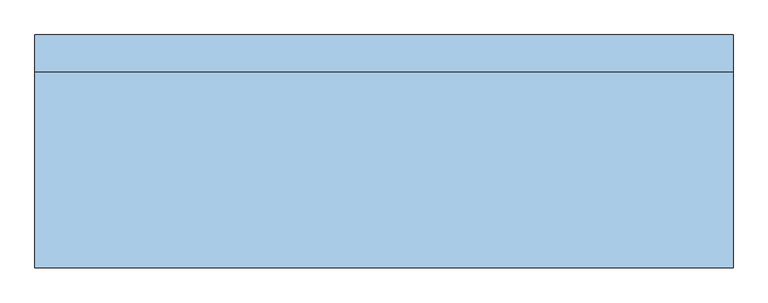
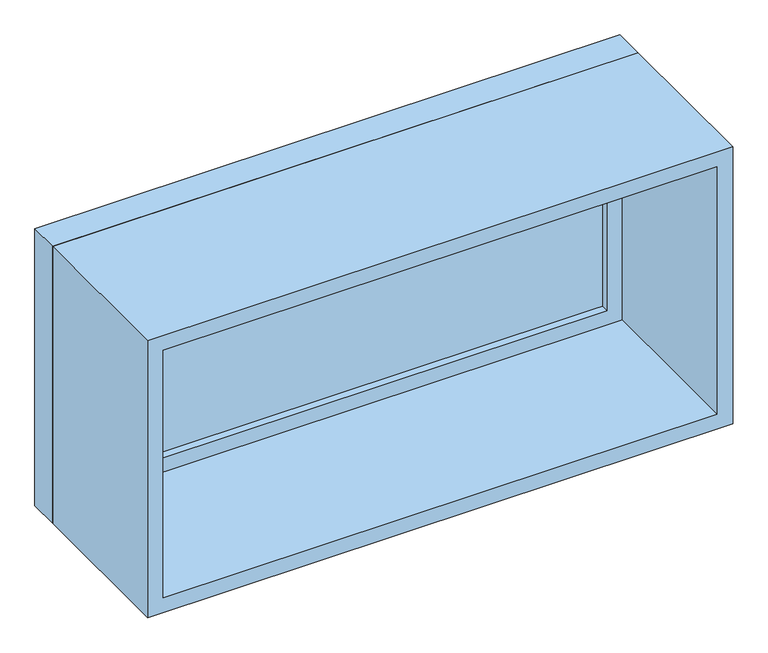
"""IFC4 building model written with IfcOpenShell, lengths in millimetres: window geometry, Фиксированные : 1200х600."""

from ifc_helpers import new_model, si_unit, frame, origin, place, context, project, spatial, polyline, outline, extrude, source, transform, mapped, element, save


def window_762fb1d9(model_context):
    return source(origin(), model_context, "Body", "SweptSolid", [
        extrude(outline(polyline([(-537.0, 178.0), (537.0, 178.0), (537.0, 166.0), (-537.0, 166.0), (-537.0, 178.0)])), frame((0.0, 0.0, 978.0), z_axis=(0.0, 0.0, 1.0), x_axis=(1.0, 0.0, 0.0)), (0.0, 0.0, 1.0), 474.0),
        extrude(outline(polyline([(1496.0, -581.0), (934.0, -581.0), (934.0, 581.0), (1496.0, 581.0), (1496.0, -581.0)]), holes=[polyline([(1452.0, -537.0), (1452.0, 537.0), (978.0, 537.0), (978.0, -537.0), (1452.0, -537.0)])]), frame((0.0, 150.0, 0.0), z_axis=(0.0, 1.0, 0.0), x_axis=(0.0, 0.0, 1.0)), (0.0, 0.0, 1.0), 44.0),
        extrude(outline(polyline([(1515.0, -600.0), (915.0, -600.0), (915.0, 600.0), (1515.0, 600.0), (1515.0, -600.0)]), holes=[polyline([(1496.0, -581.0), (1496.0, 581.0), (934.0, 581.0), (934.0, -581.0), (1496.0, -581.0)])]), frame((0.0, 150.0, 0.0), z_axis=(0.0, 1.0, 0.0), x_axis=(0.0, 0.0, 1.0)), (0.0, 0.0, 1.0), 63.0),
        extrude(outline(polyline([(1515.0, -600.0), (915.0, -600.0), (915.0, 600.0), (1515.0, 600.0), (1515.0, -600.0)]), holes=[polyline([(1483.0, -568.0), (1483.0, 568.0), (947.0, 568.0), (947.0, -568.0), (1483.0, -568.0)])]), frame((0.0, -187.0, 0.0), z_axis=(0.0, 1.0, 0.0), x_axis=(0.0, 0.0, 1.0)), (0.0, 0.0, 1.0), 337.0),
    ])


if __name__ == "__main__":
    model = new_model("IFC4")
    model_context = context("Model", 3, world=origin())
    ifc_project = project(units=[si_unit("LENGTHUNIT", "METRE", prefix="MILLI")], contexts=[model_context])
    site = spatial("IfcSite", under=ifc_project)
    building = spatial("IfcBuilding", under=site)
    placement = place(None, origin())
    window_shape = window_762fb1d9(model_context)
    element("IfcWindow", 1, ObjectType="Фиксированные : 1200х600", at=placement, inside=building, context=model_context, shape_type="MappedRepresentation", body=[
        mapped(window_shape, transform((0.0, 0.0, 0.0), x_axis=(1.0, 0.0, 0.0), y_axis=(0.0, 1.0, 0.0), z_axis=(0.0, 0.0, 1.0))),
    ])
    save(model, "model.ifc")

# Revit data of these elements
# Type "Фиксированные : 1200х600"
#   Type Mark = "19"
#   Construction Type Id = "GSP4R"
#   Analytic Construction = "Одинарное остекление стеклами Пилкингтон - 1/8 дюйма"
#   Visual Light Transmittance = 0.9
#   Solar Heat Gain Coefficient = 0.78
#   Heat Transfer Coefficient (U) = 3.6886 W/(m²·K)
#   Height = 600 mm
#   Высота подоконника по умолчанию = 915 mm
#   Width = 1200 mm
#   Вставка окна = 19 mm
#   Наружный материал каркаса = Переплет
#   Внутренний материал каркаса = Переплет
#   Материал оконного стекла = Стекло
#   Переплет = Переплет
#   Wall Closure = (empty or 0)
# Element 1 (IfcWindow, "Фиксированные : 1200х600")
#   Materials on its faces: "Переплет", "Стекло"
# Materials
#   "Переплет": class "Древесина", colour RGB 224 178 126, transparency 0, Cost = 0
#   "Стекло": class "Стекло", colour RGB 0 128 192, transparency 0.9, Description = "Известково-натриевое стекло", Cost = 0
